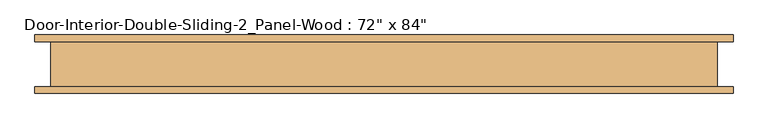
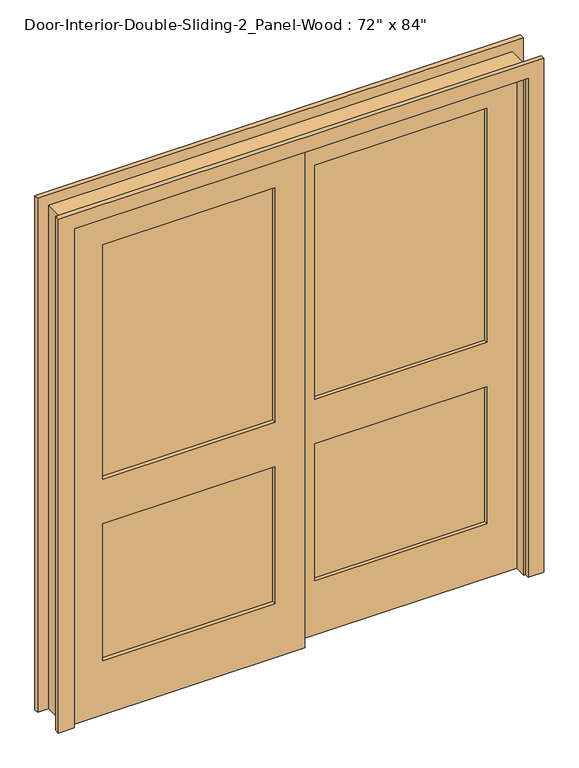
"""IFC4 building model written with IfcOpenShell, lengths in millimetres: door geometry."""

from ifc_helpers import new_model, si_unit, frame, origin, place, context, project, spatial, polyline, outline, extrude, source, transform, mapped, element, save


def door_670f2e89(model_context):
    return source(origin(), model_context, "Body", "SweptSolid", [
        extrude(outline(polyline([(793.75, 24.3416667), (793.75, 7.4083333), (95.25, 7.4083333), (95.25, 24.3416667), (793.75, 24.3416667)])), frame((0.0, 0.0, 1009.65), z_axis=(0.0, 0.0, 1.0), x_axis=(1.0, 0.0, 0.0)), (0.0, 0.0, 1.0), 1004.8875),
        extrude(outline(polyline([(793.75, 24.3416667), (793.75, 7.4083333), (95.25, 7.4083333), (95.25, 24.3416667), (793.75, 24.3416667)])), frame((0.0, 0.0, 231.775), z_axis=(0.0, 0.0, 1.0), x_axis=(1.0, 0.0, 0.0)), (0.0, 0.0, 1.0), 587.375),
        extrude(outline(polyline([(2133.6, -25.4), (0.0, -25.4), (0.0, 914.4), (2133.6, 914.4), (2133.6, -25.4)]), holes=[polyline([(2014.5375, 95.25), (2014.5375, 793.75), (1009.65, 793.75), (1009.65, 95.25), (2014.5375, 95.25)]), polyline([(819.15, 95.25), (819.15, 793.75), (231.775, 793.75), (231.775, 95.25), (819.15, 95.25)])]), frame((0.0, -9.525, 0.0), z_axis=(0.0, 1.0, 0.0), x_axis=(0.0, 0.0, 1.0)), (0.0, 0.0, 1.0), 50.8),
        extrude(outline(polyline([(-95.25, -26.4583333), (-95.25, -43.3916667), (-793.75, -43.3916667), (-793.75, -26.4583333), (-95.25, -26.4583333)])), frame((0.0, 0.0, 1009.65), z_axis=(0.0, 0.0, 1.0), x_axis=(1.0, 0.0, 0.0)), (0.0, 0.0, 1.0), 1004.8875),
        extrude(outline(polyline([(-95.25, -26.4583333), (-95.25, -43.3916667), (-793.75, -43.3916667), (-793.75, -26.4583333), (-95.25, -26.4583333)])), frame((0.0, 0.0, 231.775), z_axis=(0.0, 0.0, 1.0), x_axis=(1.0, 0.0, 0.0)), (0.0, 0.0, 1.0), 587.375),
        extrude(outline(polyline([(2133.6, -914.4), (0.0, -914.4), (0.0, 25.4), (2133.6, 25.4), (2133.6, -914.4)]), holes=[polyline([(2014.5375, -793.75), (2014.5375, -95.25), (1009.65, -95.25), (1009.65, -793.75), (2014.5375, -793.75)]), polyline([(819.15, -793.75), (819.15, -95.25), (231.775, -95.25), (231.775, -793.75), (819.15, -793.75)])]), frame((0.0, -60.325, 0.0), z_axis=(0.0, 1.0, 0.0), x_axis=(0.0, 0.0, 1.0)), (0.0, 0.0, 1.0), 50.8),
        extrude(outline(polyline([(0.0, 939.8), (2159.0, 939.8), (2159.0, -939.8), (0.0, -939.8), (0.0, -914.4), (2133.6, -914.4), (2133.6, 914.4), (0.0, 914.4), (0.0, 939.8)])), frame((0.0, -60.325, 0.0), z_axis=(0.0, 1.0, 0.0), x_axis=(0.0, 0.0, 1.0)), (0.0, 0.0, 1.0), 127.0),
        extrude(outline(polyline([(0.0, 984.25), (2203.45, 984.25), (2203.45, -984.25), (0.0, -984.25), (0.0, -920.75), (2139.95, -920.75), (2139.95, 920.75), (0.0, 920.75), (0.0, 984.25)])), frame((0.0, 66.675, 0.0), z_axis=(0.0, 1.0, 0.0), x_axis=(0.0, 0.0, 1.0)), (0.0, 0.0, 1.0), 19.05),
        extrude(outline(polyline([(0.0, 984.25), (2203.45, 984.25), (2203.45, -984.25), (0.0, -984.25), (0.0, -920.75), (2139.95, -920.75), (2139.95, 920.75), (0.0, 920.75), (0.0, 984.25)])), frame((0.0, -79.375, 0.0), z_axis=(0.0, 1.0, 0.0), x_axis=(0.0, 0.0, 1.0)), (0.0, 0.0, 1.0), 19.05),
    ])


if __name__ == "__main__":
    model = new_model("IFC4")
    model_context = context("Model", 3, world=origin())
    ifc_project = project(units=[si_unit("LENGTHUNIT", "METRE", prefix="MILLI")], contexts=[model_context])
    site = spatial("IfcSite", under=ifc_project)
    building = spatial("IfcBuilding", under=site)
    placement = place(None, origin())
    door_shape = door_670f2e89(model_context)
    element("IfcDoor", 1, ObjectType="Door-Interior-Double-Sliding-2_Panel-Wood : 72\" x 84\"", at=placement, inside=building, context=model_context, shape_type="MappedRepresentation", body=[
        mapped(door_shape, transform((0.0, 0.0, 0.0), x_axis=(1.0, 0.0, 0.0), y_axis=(0.0, 1.0, 0.0), z_axis=(0.0, 0.0, 1.0))),
    ])
    save(model, "model.ifc")

# Revit data of these elements
# Type "Door-Interior-Double-Sliding-2_Panel-Wood : 72\" x 84\""
#   Type Mark = "8"
#   Assembly Code = "C1020"
#   Analytic Construction = "Wooden"
#   Top Rail = 0' - 4 11/16"
#   Thickness = 0' - 2"
#   Thermal Resistance (R) = 2.5876 (h·ft²·°F)/BTU
#   Stiles = 0' - 4 3/4"
#   Rough Width = 6' - 2"
#   Rough Height = 7' - 1"
#   Lock Rail = 0' - 7 1/2"
#   Heat Transfer Coefficient (U) = 0.3865 BTU/(h·ft²·°F)
#   Bottom Rail = 0' - 9 1/8"
#   Height = 7' - 0"
#   Width = 6' - 0"
#   Define Thermal Properties by = 1
#   Trim Material = Cherry
#   Panel Material = Cherry
#   Frame Material = Door - Frame
#   Visual Light Transmittance = 0
#   Solar Heat Gain Coefficient = 0
#   Function = (empty or 0)
#   Wall Closure = (empty or 0)
# Element 1 (IfcDoor, "Door-Interior-Double-Sliding-2_Panel-Wood : 72\" x 84\"")
#   Materials on its faces: "Cherry", "Door - Frame"
# Materials
#   "Cherry": class "Wood", colour RGB 157 77 38, transparency 0, Description = "Prunus Serotina", Cost = 0
#   "Door - Frame": class "Unassigned", colour RGB 118 70 51, transparency 0
